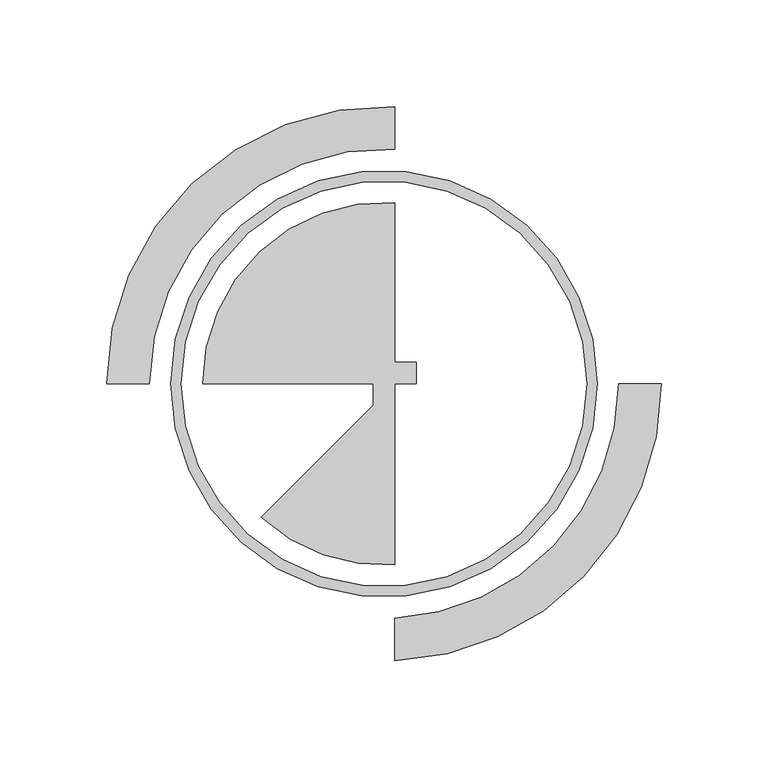
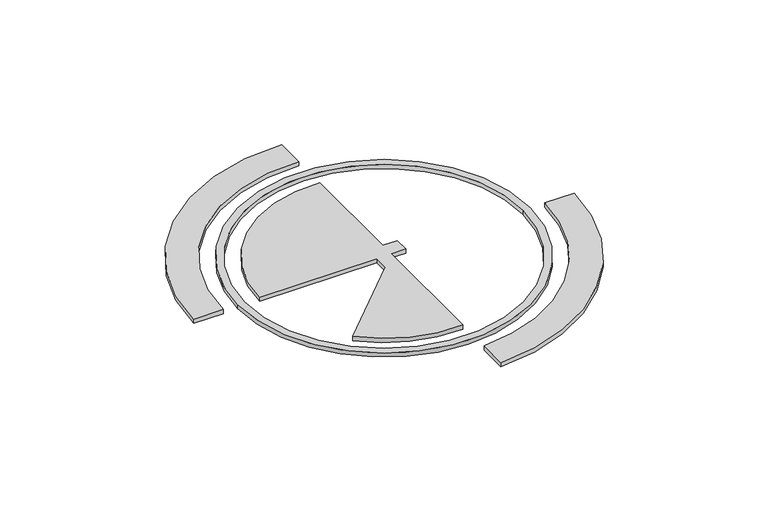
"""IFC4 building model written with IfcOpenShell, lengths in millimetres: proxy geometry, TSP Downlighter For Garage Door : TSP Downlighter For Garage Door."""

from ifc_helpers import new_model, si_unit, point, frame_2d, origin, origin_with_axes, place, context, project, spatial, polyline, circle_curve, trimmed, segment, composite_curve, outline, extrude, source, transform, mapped, element, save


def electrical_fixtures_56a16409(model_context):
    return source(origin(), model_context, "Body", "SweptSolid", [
        extrude(outline(composite_curve([segment(trimmed(circle_curve(frame_2d((-5.0, 0.0)), 100.0), [point((-105.0, 0.0))], [point((95.0, 0.0))], False, "CARTESIAN"), True, "CONTINUOUS"), segment(trimmed(circle_curve(frame_2d((-5.0, 0.0)), 100.0), [point((95.0, 0.0))], [point((-105.0, 0.0))], False, "CARTESIAN"), True, "CONTINUOUS")], self_intersect=False), holes=[composite_curve([segment(trimmed(circle_curve(frame_2d((-5.0, 0.0)), 95.0), [point((-100.0, 0.0))], [point((90.0, 0.0))], True, "CARTESIAN"), True, "CONTINUOUS"), segment(trimmed(circle_curve(frame_2d((-5.0, 0.0)), 95.0), [point((90.0, 0.0))], [point((-100.0, 0.0))], True, "CARTESIAN"), True, "CONTINUOUS")], self_intersect=False)]), origin_with_axes(), (0.0, 0.0, 1.0), 3.0),
        extrude(outline(composite_curve([segment(trimmed(circle_curve(frame_2d((-5.0, 0.0)), 85.0), [point((-90.0, 0.0))], [point((0.0, 84.8528137))], False, "CARTESIAN"), True, "CONTINUOUS"), segment(polyline([(0.0, 84.8528137), (0.0, 10.0), (10.0, 10.0), (10.0, 0.0), (0.0, 0.0), (0.0, -84.8528137)]), True, "CONTINUOUS"), segment(trimmed(circle_curve(frame_2d((-5.0, 0.0)), 85.0), [point((0.0, -84.8528137))], [point((-62.5520607, -62.5520607))], False, "CARTESIAN"), True, "CONTINUOUS"), segment(polyline([(-62.5520607, -62.5520607), (-10.0, -10.0), (-10.0, 0.0), (-90.0, 0.0)]), True, "CONTINUOUS")], self_intersect=False)), origin_with_axes(), (0.0, 0.0, 1.0), 3.0),
        extrude(outline(composite_curve([segment(trimmed(circle_curve(frame_2d((-5.0, 0.0)), 110.0), [point((0.0, 109.8863049))], [point((-115.0, 0.0))], True, "CARTESIAN"), True, "CONTINUOUS"), segment(polyline([(-115.0, 0.0), (-135.0, 0.0)]), True, "CONTINUOUS"), segment(trimmed(circle_curve(frame_2d((-5.0, 0.0)), 130.0), [point((-135.0, 0.0))], [point((0.0, 129.9038106))], False, "CARTESIAN"), True, "CONTINUOUS"), segment(polyline([(0.0, 129.9038106), (0.0, 109.8863049)]), True, "CONTINUOUS")], self_intersect=False)), origin_with_axes(), (0.0, 0.0, 1.0), 3.0),
        extrude(outline(composite_curve([segment(trimmed(circle_curve(frame_2d((-5.0, 0.0)), 110.0), [point((0.0, -109.8863049))], [point((105.0, 0.0))], True, "CARTESIAN"), True, "CONTINUOUS"), segment(polyline([(105.0, 0.0), (125.0, 0.0)]), True, "CONTINUOUS"), segment(trimmed(circle_curve(frame_2d((-5.0, 0.0)), 130.0), [point((125.0, 0.0))], [point((0.0, -129.9038106))], False, "CARTESIAN"), True, "CONTINUOUS"), segment(polyline([(0.0, -129.9038106), (0.0, -109.8863049)]), True, "CONTINUOUS")], self_intersect=False)), origin_with_axes(), (0.0, 0.0, 1.0), 3.0),
    ])


if __name__ == "__main__":
    model = new_model("IFC4")
    model_context = context("Model", 3, world=origin())
    ifc_project = project(units=[si_unit("LENGTHUNIT", "METRE", prefix="MILLI")], contexts=[model_context])
    site = spatial("IfcSite", under=ifc_project)
    building = spatial("IfcBuilding", under=site)
    placement = place(None, origin())
    electrical_fixtures_shape = electrical_fixtures_56a16409(model_context)
    element("IfcBuildingElementProxy", 1, Name="TSP Downlighter For Garage Door : TSP Downlighter For Garage Door", ObjectType="TSP Downlighter For Garage Door : TSP Downlighter For Garage Door", at=placement, inside=building, context=model_context, shape_type="MappedRepresentation", body=[
        mapped(electrical_fixtures_shape, transform((0.0, 0.0, 0.0), x_axis=(1.0, 0.0, 0.0), y_axis=(0.0, 1.0, 0.0), z_axis=(0.0, 0.0, 1.0))),
    ])
    save(model, "model.ifc")

# Revit data of these elements
# Type "TSP Downlighter For Garage Door : TSP Downlighter For Garage Door"
#   Model = "TSP_ELEC220GDL"
#   Default Elevation = 0
# Element 1 (IfcBuildingElementProxy, "TSP Downlighter For Garage Door : TSP Downlighter For Garage Door")
#   Materials on its faces: "Plastic, Opaque Black"
# Materials
#   "Plastic, Opaque Black": class "Plastic", colour RGB 0 0 0, transparency 0.7, Description = "Plastic, generic, opaque black", Cost = 0
